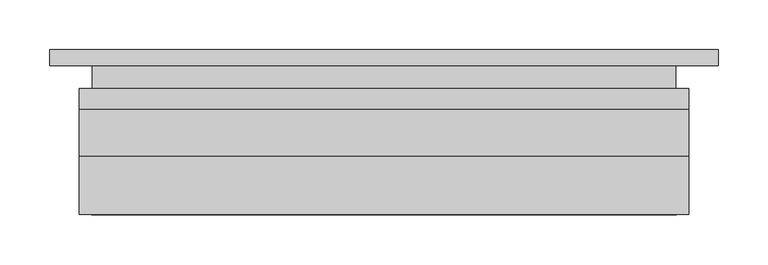
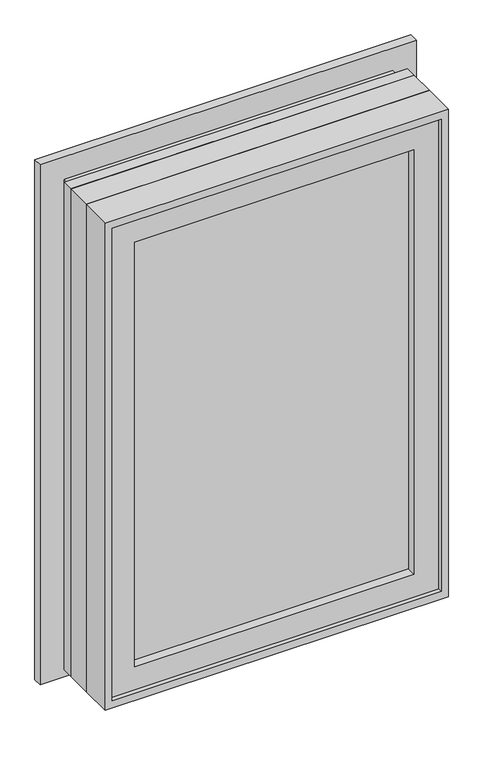
"""IFC4 building model written with IfcOpenShell, lengths in millimetres: proxy geometry, Window-Casement-Andersen-400_Series_Single : Window-Casement-Andersen-400_Series_Single."""

from ifc_helpers import new_model, si_unit, frame, origin, place, context, project, spatial, polyline, outline, extrude, faceted_brep, source, transform, mapped, element, save


def generic_models_14e9118a(model_context):
    return source(origin(), model_context, "Body", "SolidModel", [
        extrude(outline(polyline([(-248.08815, -27.8804687), (-248.08815, -12.0054687), (248.0056, -12.0054687), (248.0056, -27.8804687), (-248.08815, -27.8804687)])), frame((0.0, 0.0, 1231.9154446), z_axis=(0.0, 0.0, 1.0), x_axis=(1.0, 0.0, 0.0)), (0.0, 0.0, 1.0), 796.925),
        extrude(outline(polyline([(2074.8779446, -292.53815), (1189.0529446, -292.53815), (1189.0529446, 292.4556), (2074.8779446, 292.4556), (2074.8779446, -292.53815)]), holes=[polyline([(2028.8404446, -248.08815), (2028.8404446, 248.0056), (1231.9154446, 248.0056), (1231.9154446, -248.08815), (2028.8404446, -248.08815)])]), frame((0.0, -44.45, 0.0), z_axis=(0.0, 1.0, 0.0), x_axis=(0.0, 0.0, 1.0)), (0.0, 0.0, 1.0), 50.8),
        faceted_brep([(-276.6314, 6.35, 2060.956), (276.6314, 6.35, 2060.956), (276.6314, 57.15, 2060.956), (-276.6314, 57.15, 2060.956), (-276.6314, 6.35, 1199.769), (-276.6314, 53.2892, 1199.769), (276.6314, 53.2892, 1199.769), (276.6314, 6.35, 1199.769), (-276.6314, 57.15, 1202.53125), (-276.6314, 53.2892, 1202.53125), (276.6314, 57.15, 1202.53125), (258.7752, 57.15, 1217.2188), (258.7752, 57.15, 2040.763), (-258.7752, 57.15, 2040.763), (-258.7752, 57.15, 1217.2188), (-258.7752, 46.175563, 1236.2942), (-258.7752, 46.175563, 1225.8587599), (-258.7752, 53.3654, 1217.2188), (-258.7752, 31.75, 2040.763), (-258.7752, 31.75, 1236.2942), (258.7752, 31.75, 2040.763), (258.7752, 31.75, 1236.2942), (254.0, 31.75, 1238.25), (254.0, 31.75, 2031.603125), (-254.0, 31.75, 2031.603125), (-254.0, 31.75, 1238.25), (-254.0, 6.35, 2031.603125), (-254.0, 6.35, 1231.138), (-254.0, 13.1318, 1238.25), (254.0, 6.35, 2031.603125), (254.0, 6.35, 1231.138), (254.0, 13.1318, 1238.25), (258.7752, 53.3654, 1217.2188), (258.7752, 46.175563, 1225.8587599), (258.7752, 46.175563, 1236.2942), (276.6314, 53.2892, 1202.53125), (-277.01875, 73.9267, 2061.36875), (277.01875, 73.9267, 2061.36875), (277.01875, 53.2892, 2061.36875), (-277.01875, 53.2892, 2061.36875), (-304.8, 53.2892, 2089.15), (304.8, 53.2892, 2089.15), (304.8, 73.9267, 2089.15), (-304.8, 73.9267, 2089.15), (277.01875, 73.9267, 1202.53125), (277.01875, 53.2892, 1202.53125), (304.8, 53.2892, 1174.75), (304.8, 73.9267, 1174.75), (-277.01875, 73.9267, 1202.53125), (-277.01875, 53.2892, 1202.53125), (-304.8, 53.2892, 1174.75), (-304.8, 73.9267, 1174.75)], [[[0, 1, 2, 3]], [[4, 5, 6, 7]], [[3, 8, 9, 5, 4, 0]], [[2, 10, 8, 3], [11, 12, 13, 14]], [[15, 16, 17, 14, 13, 18, 19]], [[19, 18, 20, 21], [22, 23, 24, 25]], [[25, 24, 26, 27, 28]], [[7, 1, 0, 4], [27, 26, 29, 30]], [[31, 30, 29, 23, 22]], [[21, 20, 12, 11, 32, 33, 34]], [[1, 7, 6, 35, 10, 2]], [[25, 28, 31, 22]], [[30, 31, 28, 27]], [[15, 19, 21, 34]], [[34, 33, 16, 15]], [[33, 32, 17, 16]], [[14, 17, 32, 11]], [[12, 20, 18, 13]], [[23, 29, 26, 24]], [[36, 37, 38, 39]], [[40, 41, 42, 43]], [[37, 44, 45, 38]], [[41, 46, 47, 42]], [[44, 48, 49, 9, 8, 10, 35, 45]], [[46, 50, 51, 47]], [[39, 49, 48, 36]], [[42, 47, 51, 43], [36, 48, 44, 37]], [[43, 51, 50, 40]], [[40, 50, 46, 41], [38, 45, 35, 6, 5, 9, 49, 39]]]),
        extrude(outline(polyline([(2089.15, -304.8), (1174.75, -304.8), (1174.75, 304.8), (2089.15, 304.8), (2089.15, -304.8)]), holes=[polyline([(2060.956, -276.6314), (2060.956, 276.6314), (1199.769, 276.6314), (1199.769, -276.6314), (2060.956, -276.6314)])]), frame((0.0, 6.35, 0.0), z_axis=(0.0, 1.0, 0.0), x_axis=(0.0, 0.0, 1.0)), (0.0, 0.0, 1.0), 46.9392),
        extrude(outline(polyline([(2089.15, -304.8), (1174.75, -304.8), (1174.75, 304.8), (2089.15, 304.8), (2089.15, -304.8)]), holes=[polyline([(2074.8470554, -292.4556), (2074.8470554, 292.4556), (1189.0529446, 292.4556), (1189.0529446, -292.4556), (2074.8470554, -292.4556)])]), frame((0.0, -52.3748, 0.0), z_axis=(0.0, 1.0, 0.0), x_axis=(0.0, 0.0, 1.0)), (0.0, 0.0, 1.0), 58.7248),
        extrude(outline(polyline([(2118.51875, 334.16875), (2118.51875, -334.16875), (1142.619, -334.16875), (1142.619, 334.16875), (2118.51875, 334.16875)]), holes=[polyline([(2061.36875, 277.01875), (1199.769, 277.01875), (1199.769, -277.01875), (2061.36875, -277.01875), (2061.36875, 277.01875)])]), frame((0.0, 96.8375, 0.0), z_axis=(0.0, 1.0, 0.0), x_axis=(0.0, 0.0, 1.0)), (0.0, 0.0, 1.0), 15.875),
        extrude(outline(polyline([(2076.45, 292.1), (2076.45, -292.1), (1187.45, -292.1), (1187.45, 292.1), (2076.45, 292.1)]), holes=[polyline([(2061.36875, 277.01875), (1199.769, 277.01875), (1199.769, -277.01875), (2061.36875, -277.01875), (2061.36875, 277.01875)])]), frame((0.0, 53.18125, 0.0), z_axis=(0.0, 1.0, 0.0), x_axis=(0.0, 0.0, 1.0)), (0.0, 0.0, 1.0), 43.65625),
    ])


if __name__ == "__main__":
    model = new_model("IFC4")
    model_context = context("Model", 3, world=origin())
    ifc_project = project(units=[si_unit("LENGTHUNIT", "METRE", prefix="MILLI")], contexts=[model_context])
    site = spatial("IfcSite", under=ifc_project)
    building = spatial("IfcBuilding", under=site)
    placement = place(None, origin())
    generic_models_shape = generic_models_14e9118a(model_context)
    element("IfcBuildingElementProxy", 1, Name="Window-Casement-Andersen-400_Series_Single : Window-Casement-Andersen-400_Series_Single", ObjectType="Window-Casement-Andersen-400_Series_Single : Window-Casement-Andersen-400_Series_Single", at=placement, inside=building, context=model_context, shape_type="MappedRepresentation", body=[
        mapped(generic_models_shape, transform((0.0, 0.0, 0.0), x_axis=(1.0, 0.0, 0.0), y_axis=(0.0, 1.0, 0.0), z_axis=(0.0, 0.0, 1.0))),
    ])
    save(model, "model.ifc")

# Revit data of these elements
# Type "Window-Casement-Andersen-400_Series_Single : Window-Casement-Andersen-400_Series_Single"
#   Type Mark = "2"
#   Learn About These Parameters = "http://www.andersenwindows.com/for-professionals/cad-symbols-bim-support-window-doors/bim-support"
#   ..Jamb Condition Number 1 = "Extension Jamb Only"
#   ..Jamb Condition Number 2 = "Narrow Drywall Return"
#   ..Jamb Condition Number 3 = "Wide Drywall Return"
#   Available Grille Bar Sizes = "3/4'', 7/8'', 1 1/8'', 2 1/4''"
#   Between Glass Grille Bar Sizes = "3/4'', 1''"
#   ..Pattern Number 1 = "Colonial"
#   ..Pattern Number 2 = "Modified Colonial"
#   ..Pattern Number 3 = "Prairie"
#   ..Pattern Number 4 = "Short Fractional"
#   ..Pattern Number 5 = "Tall Fractional"
#   ..Exterior Trim Number 0 = "No Exterior Trim"
#   ..Exterior Trim Number 1 = "Brick Mould"
#   ..Exterior Trim Number 2 = "3 1/2'' Flat Casing"
#   ..Exterior Trim Number 3 = "4 1/2'' Flat Casing"
#   URL = "www.andersenwindows.com"
#   Type Comments = "Vinyl-clad wood casement window"
#   Product Documentation Link = "https://www.andersenwindows.com/windows-and-doors/windows/casement-windows/400-series-casement-window/"
#   Model = "400-Series Casement"
#   Manufacturer = "Andersen Corporation"
#   Family Version = "01.01.19"
#   Designation = "CMT"
#   Description = "Vinyl-clad wood casement window"
#   Assembly Code = "B2020100"
#   XPanelWidth = 1' - 11 1/32"
#   XPanelHeight = 2' - 10 7/8"
#   Width = 2' - 0"
#   Visual Light Transmittance = 0.48
#   Thermal Resistance (R) = 0.628713 (stored number, unit not read)
#   Solar Heat Gain Coefficient = 0.21
#   Rough Width = 2' - 0 1/2"
#   Rough Height = 3' - 0 1/2"
#   Height = 3' - 0"
#   Heat Transfer Coefficient (U) = 1.58991 (stored number, unit not read)
#   Grille Bar Size = 0' - 0 7/8"
#   xjamb S1 [instance default] = 0' - 1 23/32"
#   sill nose1 = 0' - 1 13/16"
#   sill nose 2 = 0' - 1 15/16"
#   casingS2 = 0' - 0 3/16"
#   casingS1 = 0' - 0 3/16"
#   casing4 = 0' - 4 1/4"
#   casing3 = 0' - 0 1/2"
#   casing2 = 0' - 0 7/8"
#   casing1 = 0' - 0 1/4"
#   Xjamb 2 = 0' - 0 1/2"
#   Xjamb 1 = 0' - 1 3/32"
#   Wall Thickness [instance default] = 0' - 6"
#   Wall Depth [instance default] = 0' - 4 9/16"
#   Void Offset 2 = 0' - 0"
#   Void Offset 1 = 0' - 0"
#   Void Depth [instance default] = 0' - 2 7/16"
#   VGB DLO = 0' - 5.91667"
#   TS V DLO = 2' - 7 3/8"
#   TS V Bar Length = 2' - 7 3/8"
#   TS SH DLO = 1' - 6 1/16"
#   TS HGB DLO = 0' - 9 7/8"
#   Step Jamb2 = 0' - 0 13/16"
#   Step Jamb1 = 0' - 1 1/8"
#   Sill Stop Dim [instance default] = 0' - 2 1/2"
#   SGO = 0' - 2 1/4"
#   Rough Opening Offset = 0' - 0 1/4"
#   Plan Exterior Mask 2 [instance default] = 0' - 1 3/8"
#   Plan Exterior Mask [instance default] = 0' - 1 1/16"
#   Masonry Width = 2' - 0 1/2"
#   Masonry Opening Offset = 0' - 0 1/4"
#   Masonry Height = 3' - 0 1/2"
#   JGO = 0' - 2 1/4"
#   Interior Casing Size = 0' - 2 1/4"
#   Horizontal Craftsman Bar Size = 0' - 0 7/8"
#   Head Stop Dim [instance default] = 0' - 2 17/64"
#   HGO = 0' - 2 3/8"
#   H DLO = 1' - 7 1/2"
#   Default Sill Height = 3' - 10"
#   Coarse Plan [instance default] = 0' - 4 9/16"
#   TFL = 2
#   TFB = 1
#   LWide = 3
#   Fractional Lights Wide = 3
#   Fractional Lights High = 5
#   Enter Jamb Condition = 1
#   Interior Casing = yes
#   Enter Pattern Number = 1
#   . . Lights Wide = 3
#   . . Lights High = 3
#   Extension Jamb = yes
#   Enter Exterior Trim Number = 0
#   Interior Grille Bar = yes
#   Exterior Grille Bar = yes
#   Between Glass Grille Bar = yes
#   xjamb Visibility [instance default] = yes
#   VeriLock Sensor [instance default] = no
#   V Bars = 2
#   TS S V = no
#   TS S H Craftsman = no
#   TS S H = no
#   TS M V = yes
#   TS M H = yes
#   TS H Bars = 2
#   Step Visibility = no
#   Push Out Stop Visibility [instance default] = no
#   Plan Exterior Mask Visibility [instance default] = yes
#   Nail Fin Visibility = yes
#   Interior Trim Visibility = yes
#   Crank Out Stop Visibility [instance default] = yes
#   Casing Visibility = no
#   Bar Center Line = 2
#   Glazing Material = DOUBLE HUNG WINDOWS
#   Exterior Unit Finish = Vinyl - Andersen - White
#   Interior Material = Wood - Andersen - Pine
#   Exterior Trim Finish = Fibrex Composite - Andersen - White
#   Between Glass Grille Bar Finish = Stainless Steel - Andersen - Standard
#   Wall Closure = (empty or 0)
# Element 1 (IfcBuildingElementProxy, "Window-Casement-Andersen-400_Series_Single : Window-Casement-Andersen-400_Series_Single")
#   Wall Thickness = 0' - 7 5/8"
#   Void Depth = 0' - 4 1/16"
#   Plan Exterior Mask 2 = 0' - 3"
#   Materials on its faces: "Wood - Andersen - Pine", "Vinyl - Andersen - White", "DOUBLE HUNG WINDOWS"
# Materials
#   "DOUBLE HUNG WINDOWS": class "Glass", colour RGB 236 240 239, transparency 0.85, Cost = 0
#   "Vinyl - Andersen - White": class "Plastic", colour RGB 241 238 228, transparency 0, Description = "White vinyl finish", Cost = 0
#   "Wood - Andersen - Pine": class "Wood", colour RGB 235 199 148, transparency 0, Description = "Pinus Echinata", Cost = 0
#   "Fibrex Composite - Andersen - White": class "Plastic", colour RGB 241 238 228, transparency 0, Manufacturer = "Andersen", Description = "Wood fiber and thermoplastic polymer composite material", Cost = 0
#   "Stainless Steel - Andersen - Standard": class "Metal", colour RGB 149 149 150, transparency 0, Cost = 0
